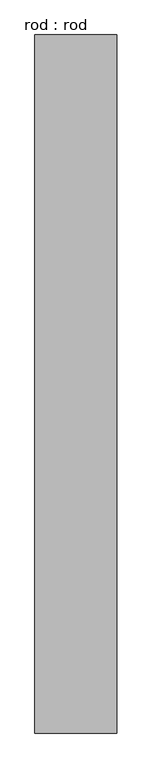
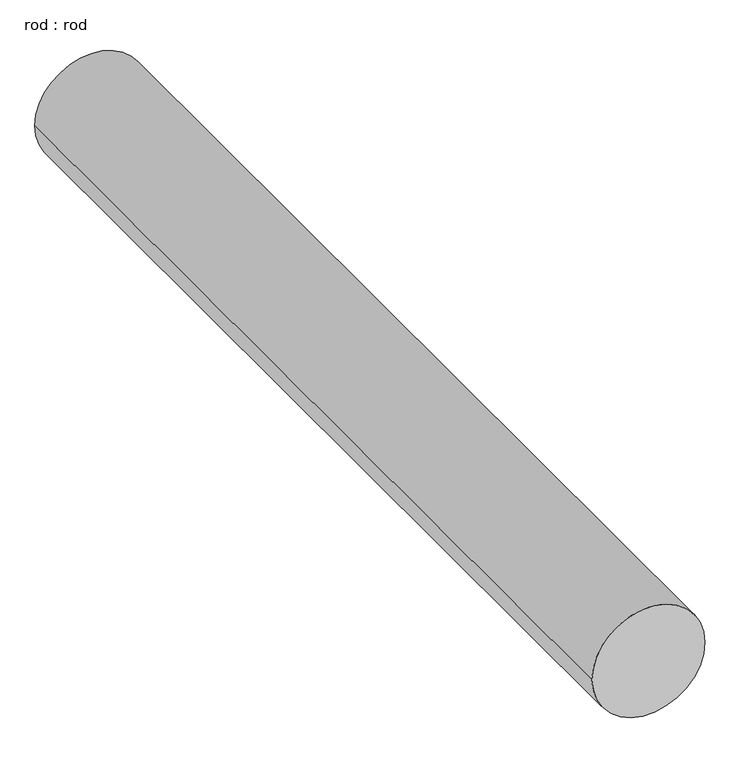
"""IFC4 building model written with IfcOpenShell, lengths in millimetres: proxy geometry, rod : rod."""

from ifc_helpers import new_model, si_unit, point, frame, frame_2d, origin, place, context, project, spatial, circle_curve, trimmed, segment, composite_curve, outline, extrude, source, transform, mapped, element, save


def rod_rod_1238732b(model_context):
    return source(origin(), model_context, "Body", "SweptSolid", [
        extrude(outline(composite_curve([segment(trimmed(circle_curve(frame_2d((0.0108462, 0.0)), 200.0), [point((0.0108462, 200.0))], [point((0.0108462, -200.0))], False, "CARTESIAN"), True, "CONTINUOUS"), segment(trimmed(circle_curve(frame_2d((0.0108462, 0.0)), 200.0), [point((0.0108462, -200.0))], [point((0.0108462, 200.0))], False, "CARTESIAN"), True, "CONTINUOUS")], self_intersect=False)), frame((0.0, 2383.8000439, 0.0), z_axis=(0.0, 1.0, 0.0), x_axis=(0.0, 0.0, 1.0)), (0.0, 0.0, 1.0), 3417.8571429),
    ])


if __name__ == "__main__":
    model = new_model("IFC4")
    model_context = context("Model", 3, world=origin())
    ifc_project = project(units=[si_unit("LENGTHUNIT", "METRE", prefix="MILLI")], contexts=[model_context])
    site = spatial("IfcSite", under=ifc_project)
    building = spatial("IfcBuilding", under=site)
    placement = place(None, origin())
    rod_rod_shape = rod_rod_1238732b(model_context)
    element("IfcBuildingElementProxy", 1, Name="rod : rod", ObjectType="rod : rod", at=placement, inside=building, context=model_context, shape_type="MappedRepresentation", body=[
        mapped(rod_rod_shape, transform((0.0, 0.0, 0.0), x_axis=(1.0, 0.0, 0.0), y_axis=(0.0, 1.0, 0.0), z_axis=(0.0, 0.0, 1.0))),
    ])
    save(model, "model.ifc")

# Revit data of these elements
# Type "rod : rod"
#   Default Elevation = 0
